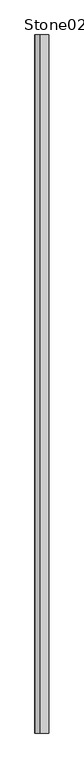
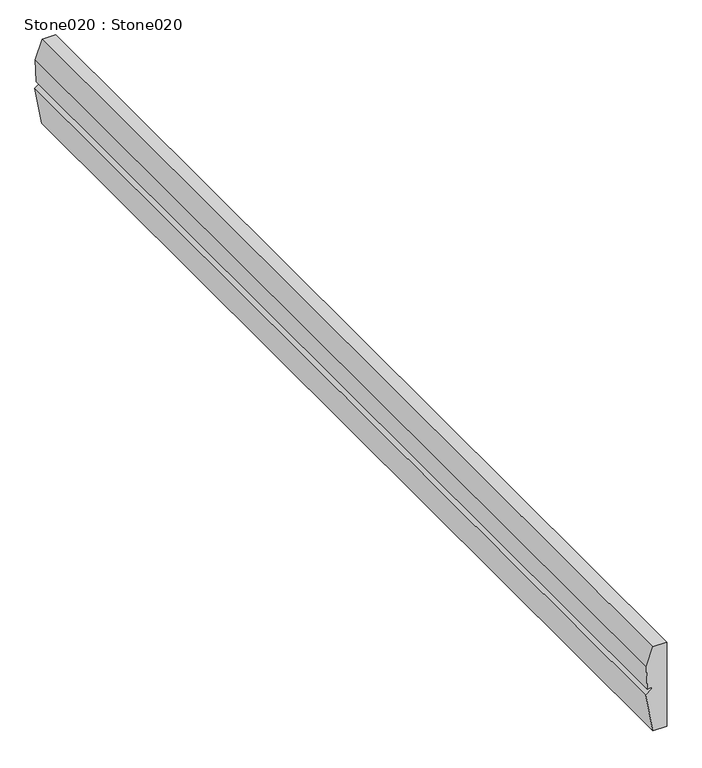
"""IFC4 building model written with IfcOpenShell, lengths in millimetres: proxy geometry, Stone020 : Stone020."""

from ifc_helpers import new_model, si_unit, frame, origin, place, context, project, spatial, polyline, outline, extrude, source, transform, mapped, element, save


def stone020_stone020_adb5f35a(model_context):
    return source(origin(), model_context, "Body", "SweptSolid", [
        extrude(outline(polyline([(32956.2773438, -10292.2685547), (32920.484375, -10304.7431641), (32875.1640625, -10303.0371094), (32876.1835938, -10294.5625), (32872.7304688, -10294.0849609), (32863.9453125, -10305.7998047), (32788.7148438, -10292.7705078), (32788.7148438, -10266.1494141), (32956.2773438, -10266.1494141), (32956.2773438, -10292.2685547)])), frame((0.0, 7982.1531721, 0.0), z_axis=(0.0, 1.0, 0.0), x_axis=(0.0, 0.0, 1.0)), (0.0, 0.0, 1.0), 2000.0),
    ])


if __name__ == "__main__":
    model = new_model("IFC4")
    model_context = context("Model", 3, world=origin())
    ifc_project = project(units=[si_unit("LENGTHUNIT", "METRE", prefix="MILLI")], contexts=[model_context])
    site = spatial("IfcSite", under=ifc_project)
    building = spatial("IfcBuilding", under=site)
    placement = place(None, origin())
    stone020_stone020_shape = stone020_stone020_adb5f35a(model_context)
    element("IfcBuildingElementProxy", 1, Name="Stone020 : Stone020", ObjectType="Stone020 : Stone020", at=placement, inside=building, context=model_context, shape_type="MappedRepresentation", body=[
        mapped(stone020_stone020_shape, transform((0.0, 0.0, 0.0), x_axis=(1.0, 0.0, 0.0), y_axis=(0.0, 1.0, 0.0), z_axis=(0.0, 0.0, 1.0))),
    ])
    save(model, "model.ifc")

# Revit data of these elements
# Type "Stone020 : Stone020"
#   NameOverride = "Stone020"
# Element 1 (IfcBuildingElementProxy, "Stone020 : Stone020")
#   Materials on its faces: "SPLIT FACE STONE"
# Materials
#   "SPLIT FACE STONE": class "Unassigned", colour RGB 205 195 181, transparency 0, Cost = 0
